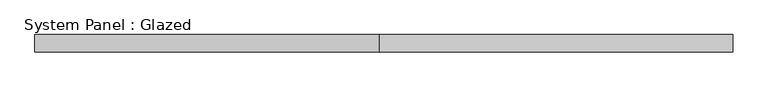
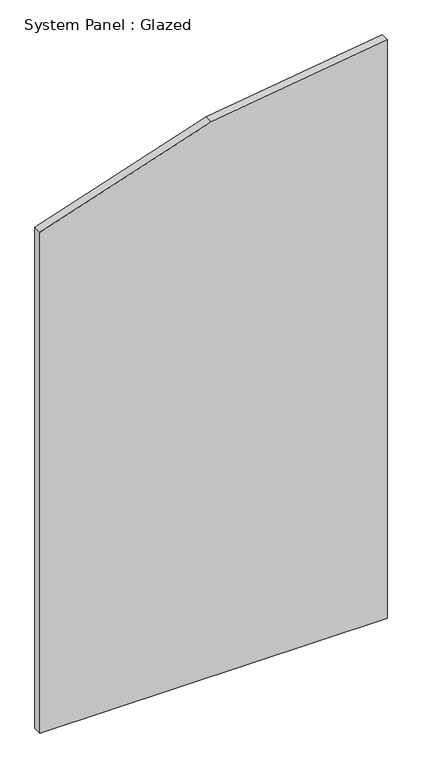
"""IFC4 building model written with IfcOpenShell, lengths in millimetres: plate geometry, System Panel : Glazed."""

import ifcopenshell
import ifcopenshell.guid

model = None  # the IFC model being written
_history = None  # IfcOwnerHistory: only IFC2X3 demands one
_inside = {}  # id of a spatial element -> (the spatial element, [elements in it])
_under = {}  # id of a project, library or spatial element -> (it, [spatial elements below it])
_declared = {}  # id of a project -> (the project, [libraries it declares])
_typed = {}  # id of a type object -> (the type object, [elements of that type])
_made_of = {}  # id of a material, layer set ... -> (it, [elements and type objects made of it])


def new_model(schema):
    """Start an empty IFC model of exactly this schema.

    Asked for "IFC4X3", IfcOpenShell would pick the latest addendum, in which some entities
    have other attributes; the version numbers below select the first issue.
    IFC2X3 requires an IfcOwnerHistory on every rooted entity: one is made here for all.
    """
    global model, _history
    if schema == "IFC4X3":
        model = ifcopenshell.file(schema_version=(4, 3, 0, 0))
    else:
        model = ifcopenshell.file(schema=schema)
    _inside.clear()
    _under.clear()
    _declared.clear()
    _typed.clear()
    _made_of.clear()
    _history = None
    if model.schema == "IFC2X3":
        org = make("IfcOrganization", Name="unknown")
        user = make(
            "IfcPersonAndOrganization",
            ThePerson=make("IfcPerson", FamilyName="unknown"),
            TheOrganization=org,
        )
        app = make(
            "IfcApplication",
            ApplicationDeveloper=org,
            Version="unknown",
            ApplicationFullName="unknown",
            ApplicationIdentifier="unknown",
        )
        _history = make(
            "IfcOwnerHistory",
            OwningUser=user,
            OwningApplication=app,
            ChangeAction="ADDED",
            CreationDate=0,
        )
    return model


def make(cls, **values):
    """One entity of the class cls with the attributes given. An attribute that is None is left unset."""
    return model.create_entity(
        cls, **{name: value for name, value in values.items() if value is not None}
    )


def rooted(cls, **values):
    """An entity with a GlobalId (a new one), such as an element, a storey or a relation."""
    return make(cls, GlobalId=ifcopenshell.guid.new(), OwnerHistory=_history, **values)


def si_unit(unit_type, name, prefix=None):
    """IfcSIUnit, for example si_unit("LENGTHUNIT", "METRE", prefix="MILLI")."""
    return make("IfcSIUnit", UnitType=unit_type, Prefix=prefix, Name=name)


def assignment(units):
    """IfcUnitAssignment: the units of a project."""
    return None if units is None else make("IfcUnitAssignment", Units=units)


def point(xyz):
    """IfcCartesianPoint."""
    return None if xyz is None else make("IfcCartesianPoint", Coordinates=xyz)


def direction(xyz):
    """IfcDirection."""
    return None if xyz is None else make("IfcDirection", DirectionRatios=xyz)


def frame(location, z_axis=None, x_axis=None):
    """IfcAxis2Placement3D, a coordinate frame: its origin and axes. An axis left out is left unset."""
    return make(
        "IfcAxis2Placement3D",
        Location=point(location),
        Axis=direction(z_axis),
        RefDirection=direction(x_axis),
    )


def origin():
    """The frame at (0, 0, 0) with its axes left unset."""
    return frame((0.0, 0.0, 0.0))


def place(relative_to, where):
    """IfcLocalPlacement: puts the frame where relative to a parent placement (None: the world)."""
    return make(
        "IfcLocalPlacement", PlacementRelTo=relative_to, RelativePlacement=where
    )


def context(
    kind, dimensions, precision=None, world=None, true_north=None, identifier=None
):
    """IfcGeometricRepresentationContext, for example the 3D "Model" context."""
    return make(
        "IfcGeometricRepresentationContext",
        ContextIdentifier=identifier,
        ContextType=kind,
        CoordinateSpaceDimension=dimensions,
        Precision=precision,
        WorldCoordinateSystem=world,
        TrueNorth=true_north,
    )


def project(units=None, contexts=None):
    """IfcProject with its units and contexts."""
    return rooted(
        "IfcProject",
        Name="project",
        RepresentationContexts=contexts,
        UnitsInContext=assignment(units),
    )


def spatial(cls, under=None, at=None, **own):
    """A site, building, storey or space (cls), placed at a placement, below another one or the project."""
    s = rooted(cls, ObjectPlacement=at, **own)
    if under is not None:
        _under.setdefault(under.id(), (under, []))[1].append(s)
    return s


def polyline(points):
    """IfcPolyline through the points."""
    return make("IfcPolyline", Points=[point(p) for p in points])


def outline(outer, holes=None, kind="AREA"):
    """IfcArbitraryClosedProfileDef: a profile drawn as a closed curve; with holes, ...WithVoids."""
    if holes is None:
        return make("IfcArbitraryClosedProfileDef", ProfileType=kind, OuterCurve=outer)
    return make(
        "IfcArbitraryProfileDefWithVoids",
        ProfileType=kind,
        OuterCurve=outer,
        InnerCurves=holes,
    )


def extrude(swept, where, along, depth):
    """IfcExtrudedAreaSolid: the profile swept, set in the frame where, extruded along a direction by depth."""
    return make(
        "IfcExtrudedAreaSolid",
        SweptArea=swept,
        Position=where,
        ExtrudedDirection=direction(along),
        Depth=depth,
    )


def shape(context_of_items, identifier, shape_type, items):
    """IfcShapeRepresentation: the items that make up one representation, for example the "Body"."""
    return make(
        "IfcShapeRepresentation",
        ContextOfItems=context_of_items,
        RepresentationIdentifier=identifier,
        RepresentationType=shape_type,
        Items=items,
    )


def source(mapping_origin, context_of_items, identifier, shape_type, items):
    """IfcRepresentationMap: a shape defined once, which mapped items show again and again."""
    return make(
        "IfcRepresentationMap",
        MappingOrigin=mapping_origin,
        MappedRepresentation=shape(context_of_items, identifier, shape_type, items),
    )


def transform(
    local_origin,
    x_axis=None,
    y_axis=None,
    z_axis=None,
    scale=None,
    scale2=None,
    scale3=None,
    uniform=True,
):
    """IfcCartesianTransformationOperator3D, or its non-uniform kind. x_axis, y_axis, z_axis: its Axis1, 2, 3."""
    if uniform:
        return make(
            "IfcCartesianTransformationOperator3D",
            Axis1=direction(x_axis),
            Axis2=direction(y_axis),
            LocalOrigin=point(local_origin),
            Scale=scale,
            Axis3=direction(z_axis),
        )
    return make(
        "IfcCartesianTransformationOperator3DnonUniform",
        Axis1=direction(x_axis),
        Axis2=direction(y_axis),
        LocalOrigin=point(local_origin),
        Scale=scale,
        Axis3=direction(z_axis),
        Scale2=scale2,
        Scale3=scale3,
    )


def mapped(mapping_source, mapping_target):
    """IfcMappedItem: shows the shape of a source again, moved by a transform."""
    return make(
        "IfcMappedItem", MappingSource=mapping_source, MappingTarget=mapping_target
    )


def made_of(thing, what):
    """Note that an element or type object is made of a material, layer set ...; save() writes the relation."""
    if what is not None:
        _made_of.setdefault(what.id(), (what, []))[1].append(thing)
    return thing


def element(
    cls,
    number,
    at=None,
    inside=None,
    cuts=None,
    type_object=None,
    material=None,
    context=None,
    identifier="Body",
    shape_type=None,
    held_by="IfcProductDefinitionShape",
    body=None,
    shapes=None,
    **own,
):
    """One element of the class cls, such as IfcWall. Its Tag is "e" and its number.

    at: its placement. inside: the storey or other place that contains it. cuts: it is an
    opening in that element (IfcRelVoidsElement). A single representation is given by context,
    identifier, shape_type and body (its items); several are given by shapes. held_by: the class
    of the entity that holds the representations. save() writes the other relations.
    """
    e = rooted(cls, Tag="e%d" % number, ObjectPlacement=at, **own)
    if body is not None:
        shapes = [shape(context, identifier, shape_type, body)]
    if shapes is not None:
        e.Representation = make(held_by, Representations=shapes)
    if inside is not None:
        _inside.setdefault(inside.id(), (inside, []))[1].append(e)
    if cuts is not None:
        rooted(
            "IfcRelVoidsElement", RelatingBuildingElement=cuts, RelatedOpeningElement=e
        )
    if type_object is not None:
        _typed.setdefault(type_object.id(), (type_object, []))[1].append(e)
    return made_of(e, material)


def aggregate(whole, parts):
    """IfcRelAggregates: a whole, such as a stair, and the parts it consists of."""
    return rooted("IfcRelAggregates", RelatingObject=whole, RelatedObjects=parts)


def save(model, path):
    """Write the relations noted so far, then the file.

    IfcRelAggregates (storeys below a building ...), IfcRelContainedInSpatialStructure (elements
    in a storey), IfcRelDefinesByType, IfcRelAssociatesMaterial and IfcRelDeclares: one each for
    every whole, place, type object, material and project.
    """
    for whole, parts in _under.values():
        aggregate(whole, parts)
    for where, things in _inside.values():
        rooted(
            "IfcRelContainedInSpatialStructure",
            RelatedElements=things,
            RelatingStructure=where,
        )
    for kind, things in _typed.values():
        rooted("IfcRelDefinesByType", RelatedObjects=things, RelatingType=kind)
    for what, things in _made_of.values():
        rooted("IfcRelAssociatesMaterial", RelatedObjects=things, RelatingMaterial=what)
    for by, libraries in _declared.values():
        rooted("IfcRelDeclares", RelatingContext=by, RelatedDefinitions=libraries)
    model.write(path)


def system_panel_glazed_6c4c7ed2(model_context):
    return source(origin(), model_context, "Body", "SweptSolid", [
        extrude(outline(polyline([(0.0, -500.0), (0.0, 500.0), (1761.3177476, 500.0), (1689.3102197, -6.2307384), (1526.050305, -500.0), (0.0, -500.0)])), frame((0.0, 24.5, 0.0), z_axis=(0.0, 1.0, 0.0), x_axis=(0.0, 0.0, 1.0)), (0.0, 0.0, 1.0), 25.0),
    ])


if __name__ == "__main__":
    model = new_model("IFC4")
    model_context = context("Model", 3, world=origin())
    ifc_project = project(units=[si_unit("LENGTHUNIT", "METRE", prefix="MILLI")], contexts=[model_context])
    site = spatial("IfcSite", under=ifc_project)
    building = spatial("IfcBuilding", under=site)
    placement = place(None, origin())
    system_panel_glazed_shape = system_panel_glazed_6c4c7ed2(model_context)
    element("IfcPlate", 1, ObjectType="System Panel : Glazed", at=placement, inside=building, context=model_context, shape_type="MappedRepresentation", body=[
        mapped(system_panel_glazed_shape, transform((0.0, 0.0, 0.0), x_axis=(1.0, 0.0, 0.0), y_axis=(0.0, 1.0, 0.0), z_axis=(0.0, 0.0, 1.0))),
    ])
    save(model, "model.ifc")

# Revit data of these elements
# Project information
#   Project Issue Date = "05/22/2020"
#   Project Status = "Project  Status"
#   Project Address = "## Street\nCity, State  Zip"
#   Project Number = "1"
# Element 1 (IfcPlate, "System Panel : Glazed")
#   Materials on its faces: "Glass"
# Materials
#   "Glass": class "Glass", colour RGB 218 227 224, transparency 0.85, Description = "Soda Lime Glass", Cost = 0
